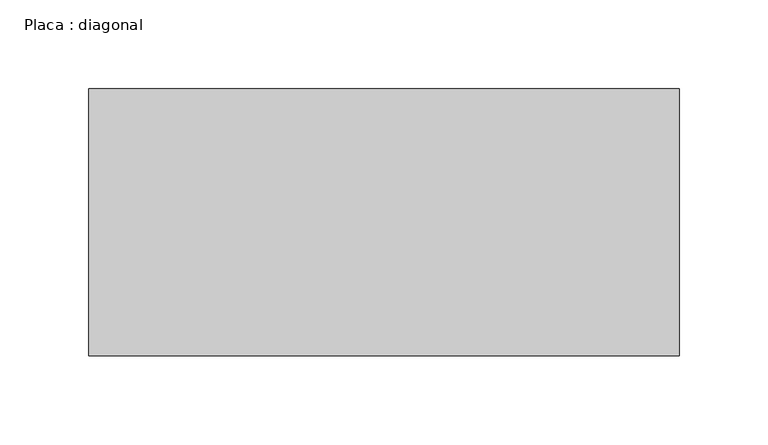
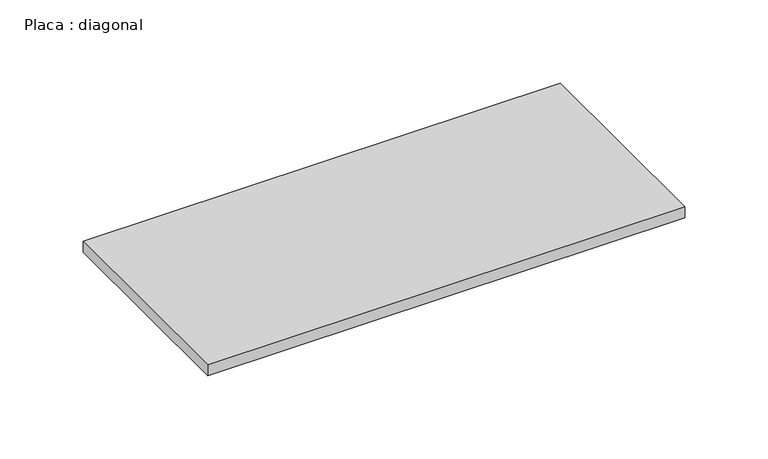
"""IFC4 building model written with IfcOpenShell, lengths in millimetres: beam geometry, Placa : diagonal."""

from ifc_helpers import new_model, si_unit, frame, origin, place, context, project, spatial, polyline, outline, extrude, source, transform, mapped, element, save


def placa_diagonal_a2e3544b(model_context):
    return source(origin(), model_context, "Body", "SweptSolid", [
        extrude(outline(polyline([(165.536904, 75.0), (165.536904, -75.0), (-166.2630935, -75.0), (-166.2630935, 75.0), (165.536904, 75.0)])), frame((0.0, 0.0, -4.0), z_axis=(0.0, 0.0, 1.0), x_axis=(1.0, 0.0, 0.0)), (0.0, 0.0, 1.0), 8.0),
    ])


if __name__ == "__main__":
    model = new_model("IFC4")
    model_context = context("Model", 3, world=origin())
    ifc_project = project(units=[si_unit("LENGTHUNIT", "METRE", prefix="MILLI")], contexts=[model_context])
    site = spatial("IfcSite", under=ifc_project)
    building = spatial("IfcBuilding", under=site)
    placement = place(None, origin())
    placa_diagonal_shape = placa_diagonal_a2e3544b(model_context)
    element("IfcBeam", 1, ObjectType="Placa : diagonal", at=placement, inside=building, context=model_context, shape_type="MappedRepresentation", body=[
        mapped(placa_diagonal_shape, transform((0.0, 0.0, 0.0), x_axis=(1.0, 0.0, 0.0), y_axis=(0.0, 1.0, 0.0), z_axis=(0.0, 0.0, 1.0))),
    ])
    save(model, "model.ifc")

# Revit data of these elements
# Type "Placa : diagonal"
#   W = 0
#   Length [instance default] = 1.50 m
#   b = 0.15 m
#   d = 0.008 m
#   A = 0 m²
#   Structural Material [instance default] = Aço, 45-345
# Element 1 (IfcBeam, "Placa : diagonal")
#   Materials on its faces: "Aço, 45-345"
# Materials
#   "Aço, 45-345": class "Metal", colour RGB 247 247 247, transparency 0, Description = "Aço 345 MPa", Cost = 0
